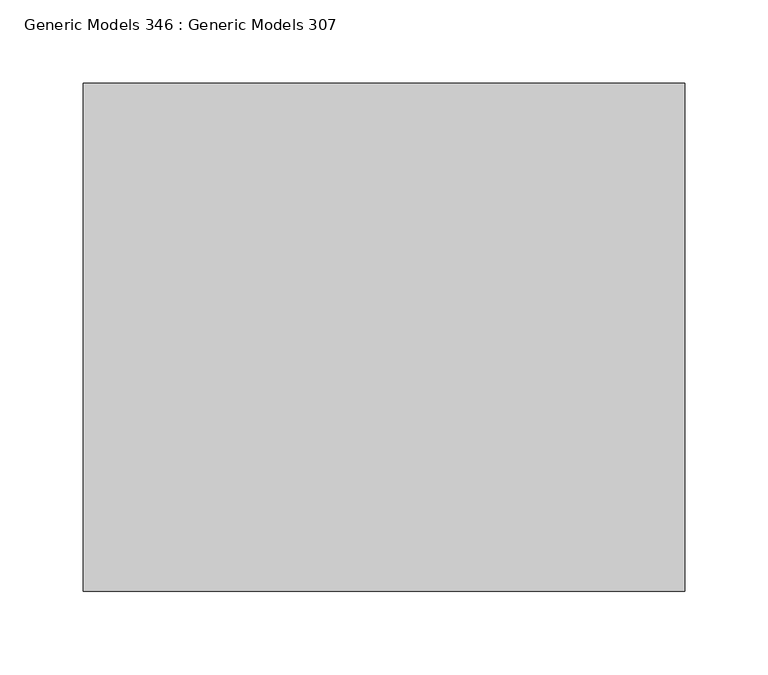
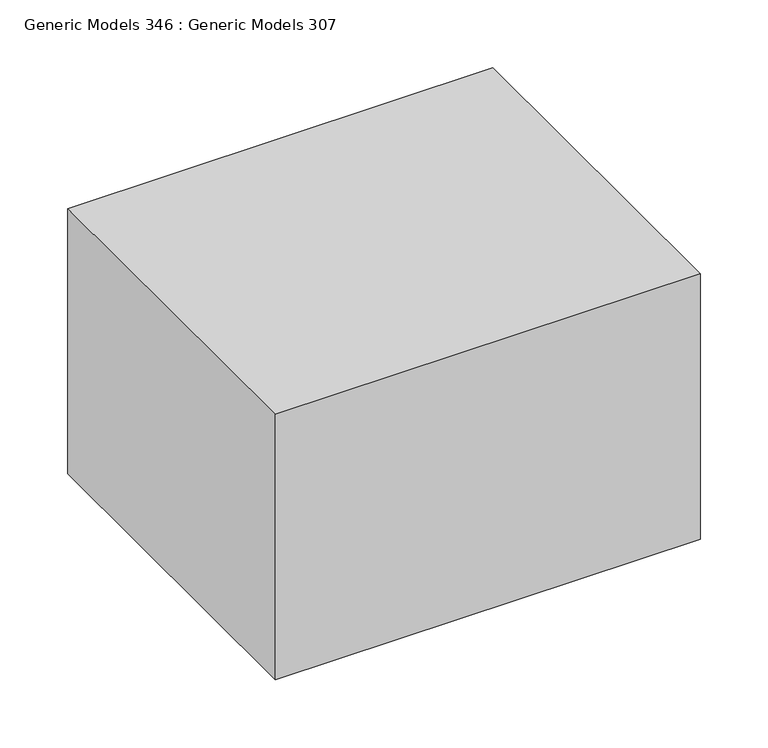
"""IFC4 building model written with IfcOpenShell, lengths in millimetres: proxy geometry, Generic Models 346 : Generic Models 307."""

from ifc_helpers import new_model, si_unit, frame, origin, place, context, project, spatial, polyline, outline, extrude, source, transform, mapped, element, save


def generic_models_346_generic_models_307_93d1f0e0(model_context):
    return source(origin(), model_context, "Body", "SweptSolid", [
        extrude(outline(polyline([(4477.3445724, 704.5309662), (4838.2221741, 704.5309662), (4838.2221741, 399.7309662), (4477.3445724, 399.7309662), (4477.3445724, 704.5309662)])), frame((0.0, 0.0, 129253.3729677), z_axis=(0.0, 0.0, 1.0), x_axis=(1.0, 0.0, 0.0)), (0.0, 0.0, 1.0), 238.1975704),
    ])


if __name__ == "__main__":
    model = new_model("IFC4")
    model_context = context("Model", 3, world=origin())
    ifc_project = project(units=[si_unit("LENGTHUNIT", "METRE", prefix="MILLI")], contexts=[model_context])
    site = spatial("IfcSite", under=ifc_project)
    building = spatial("IfcBuilding", under=site)
    placement = place(None, origin())
    generic_models_346_generic_models_307_shape = generic_models_346_generic_models_307_93d1f0e0(model_context)
    element("IfcBuildingElementProxy", 1, Name="Generic Models 346 : Generic Models 307", ObjectType="Generic Models 346 : Generic Models 307", at=placement, inside=building, context=model_context, shape_type="MappedRepresentation", body=[
        mapped(generic_models_346_generic_models_307_shape, transform((0.0, 0.0, 0.0), x_axis=(1.0, 0.0, 0.0), y_axis=(0.0, 1.0, 0.0), z_axis=(0.0, 0.0, 1.0))),
    ])
    save(model, "model.ifc")

# Revit data of these elements
# Element 1 (IfcBuildingElementProxy, "Generic Models 346 : Generic Models 307")
#   Materials on its faces: "_BATT INSUL. (R-FACTOR = R38 MIN) OVER CLASS II VAPOR RETARDER(TOWARD INTERIOR)"
# Materials
#   "_BATT INSUL. (R-FACTOR = R38 MIN) OVER CLASS II VAPOR RETARDER(TOWARD INTERIOR)": class "Generic", colour RGB 227 210 251, transparency 0, Cost = 0
